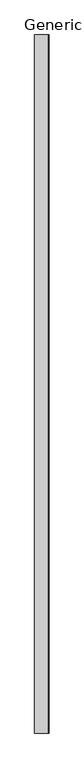
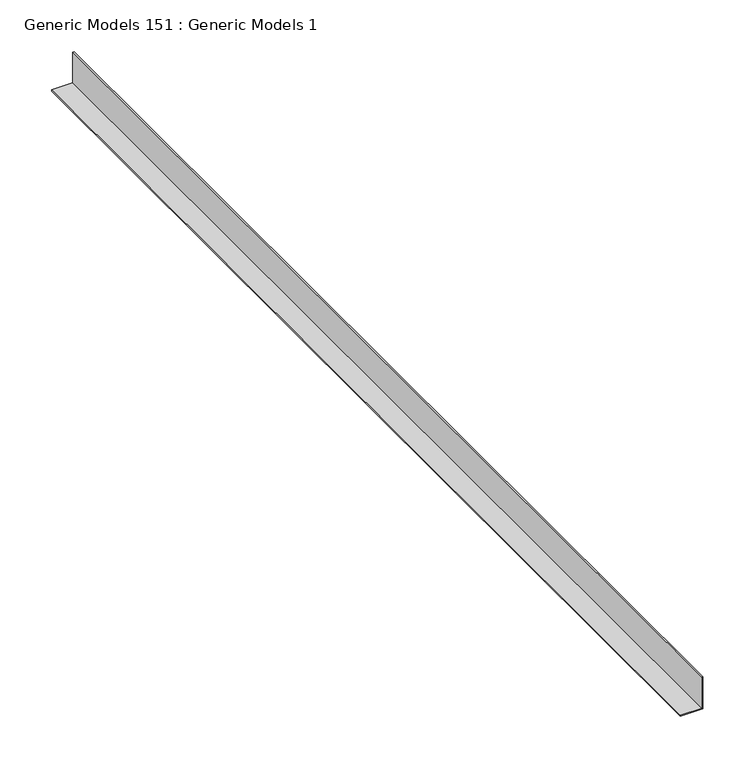
"""IFC4 building model written with IfcOpenShell, lengths in millimetres: proxy geometry, Generic Models 151 : Generic Models 1."""

from ifc_helpers import new_model, si_unit, frame, origin, place, context, project, spatial, polyline, outline, extrude, source, transform, mapped, element, save


def generic_models_151_generic_models_1_528f8659(model_context):
    return source(origin(), model_context, "Body", "SweptSolid", [
        extrude(outline(polyline([(2277.1204978, 51991.1377541), (2277.1204978, 51989.5502541), (2240.6079978, 51989.5502541), (2240.6079978, 51965.7377541), (2239.0204978, 51965.7377541), (2239.0204978, 51991.1377541), (2277.1204978, 51991.1377541)])), frame((0.0, 0.0, 0.0), z_axis=(0.0, 1.0, 0.0), x_axis=(0.0, 0.0, 1.0)), (0.0, 0.0, 1.0), 1219.2),
    ])


if __name__ == "__main__":
    model = new_model("IFC4")
    model_context = context("Model", 3, world=origin())
    ifc_project = project(units=[si_unit("LENGTHUNIT", "METRE", prefix="MILLI")], contexts=[model_context])
    site = spatial("IfcSite", under=ifc_project)
    building = spatial("IfcBuilding", under=site)
    placement = place(None, origin())
    generic_models_151_generic_models_1_shape = generic_models_151_generic_models_1_528f8659(model_context)
    element("IfcBuildingElementProxy", 1, Name="Generic Models 151 : Generic Models 1", ObjectType="Generic Models 151 : Generic Models 1", at=placement, inside=building, context=model_context, shape_type="MappedRepresentation", body=[
        mapped(generic_models_151_generic_models_1_shape, transform((0.0, 0.0, 0.0), x_axis=(1.0, 0.0, 0.0), y_axis=(0.0, 1.0, 0.0), z_axis=(0.0, 0.0, 1.0))),
    ])
    save(model, "model.ifc")

# Revit data of these elements
# Element 1 (IfcBuildingElementProxy, "Generic Models 151 : Generic Models 1")
#   Materials on its faces: "CEILING TRACK AS SCHEDULED"
# Materials
#   "CEILING TRACK AS SCHEDULED": class "Unassigned", colour RGB 210 209 208, transparency 0, Keynote = "M05121300.02", Cost = 0
